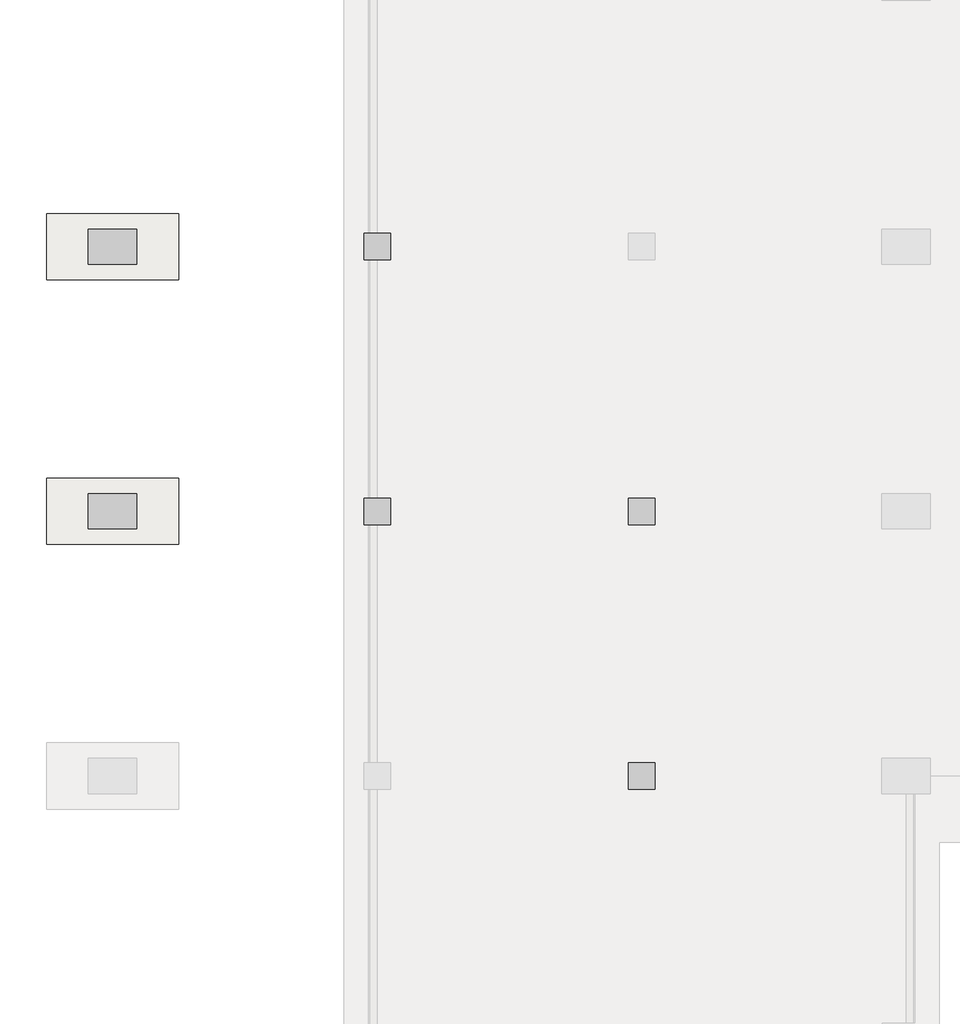
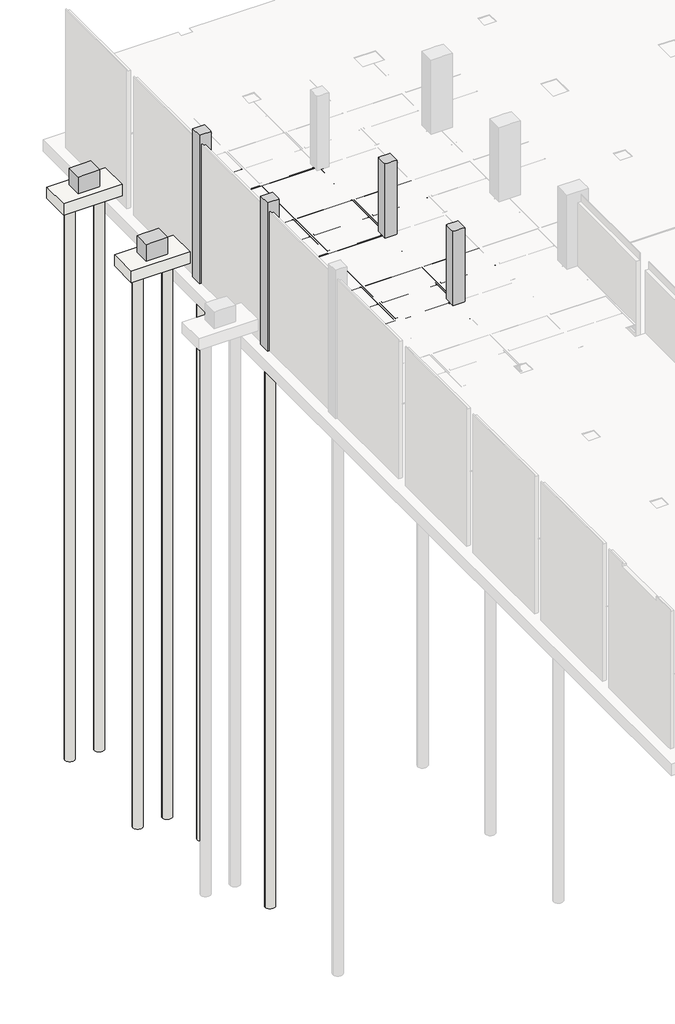
# Not in any storey, part 7 of 16: 27 beams, 8 slabs, 6 columns.
# Revit data of these elements (continued)
# Elements 30, 31, 32, 33 (IfcColumn, "RC_Column_Rectangular : H_SC_AR_S15_UG PED_Bit_600x600_BC1")
#   Comments = ""
#   hec_material3 = none
#   hec_material2 = none
#   hec_material1 = none
#   Structural Material = 00_Concrete_Reinf. Conc.
#   Phase Created = New Construction
#   Materials on its faces: "00_Concrete_Reinf. Conc."
# Elements 34, 35 (IfcSlab, "Foundation Rectangular (Non-Pile) : H_SF_AR_S18_Shallow Fdn_Bitumen_1500x3000xT600_F1")
#   Comments = ""
#   Structural Material = 00_Concrete_Reinf. Conc.
#   Phase Created = New Construction
#   Materials on its faces: "00_Concrete_Reinf. Conc."
# Elements 36, 37, 38, 39 (IfcSlab, "PILE : H_SF_AR_S19_PHC Pile_Pre-boring_D500_L30")
#   Structural Material = Concrete, Precast
#   Phase Created = New Construction
#   Materials on its faces: "Concrete, Precast"
# Elements 40, 41 (IfcSlab, "PILE : H_SF_AR_S19_PHC Pile_Pre-boring_D500_L30")
#   Structural Material = none
#   Phase Created = New Construction
# Materials
#   "Steel, 45-345": class "Metal", colour RGB 189 187 185, transparency 0, Description = "Steel 345 MPa", Cost = 0
#   "00_Concrete_Reinf. Conc.": class "Concrete", colour RGB 176 176 176, transparency 0, Description = "Reinf. Conc.", Cost = 0, Image = Concrete.Cast-In-Place.Flat.Polished.Grey.jpg
#   "Concrete, Precast": class "Concrete", colour RGB 115 116 108, transparency 0, Description = "Precast concrete", Cost = 0
